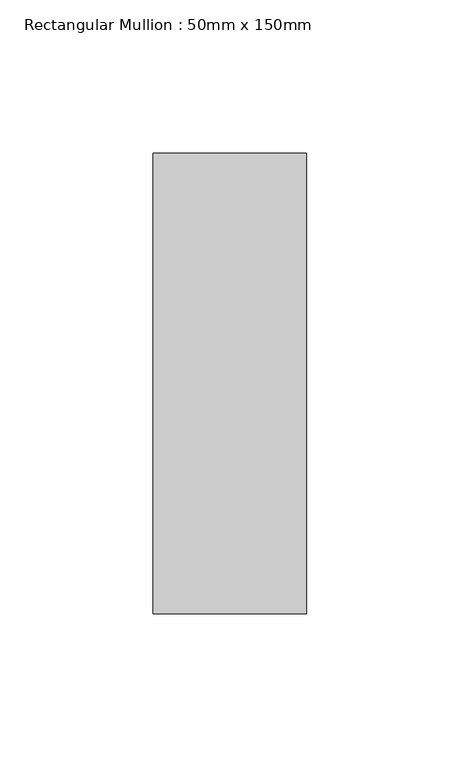
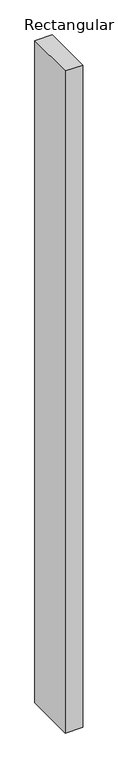
"""IFC4 building model written with IfcOpenShell, lengths in millimetres: member geometry, Rectangular Mullion : 50mm x 150mm."""

import ifcopenshell
import ifcopenshell.guid

model = None  # the IFC model being written
_history = None  # IfcOwnerHistory: only IFC2X3 demands one
_inside = {}  # id of a spatial element -> (the spatial element, [elements in it])
_under = {}  # id of a project, library or spatial element -> (it, [spatial elements below it])
_declared = {}  # id of a project -> (the project, [libraries it declares])
_typed = {}  # id of a type object -> (the type object, [elements of that type])
_made_of = {}  # id of a material, layer set ... -> (it, [elements and type objects made of it])


def new_model(schema):
    """Start an empty IFC model of exactly this schema.

    Asked for "IFC4X3", IfcOpenShell would pick the latest addendum, in which some entities
    have other attributes; the version numbers below select the first issue.
    IFC2X3 requires an IfcOwnerHistory on every rooted entity: one is made here for all.
    """
    global model, _history
    if schema == "IFC4X3":
        model = ifcopenshell.file(schema_version=(4, 3, 0, 0))
    else:
        model = ifcopenshell.file(schema=schema)
    _inside.clear()
    _under.clear()
    _declared.clear()
    _typed.clear()
    _made_of.clear()
    _history = None
    if model.schema == "IFC2X3":
        org = make("IfcOrganization", Name="unknown")
        user = make(
            "IfcPersonAndOrganization",
            ThePerson=make("IfcPerson", FamilyName="unknown"),
            TheOrganization=org,
        )
        app = make(
            "IfcApplication",
            ApplicationDeveloper=org,
            Version="unknown",
            ApplicationFullName="unknown",
            ApplicationIdentifier="unknown",
        )
        _history = make(
            "IfcOwnerHistory",
            OwningUser=user,
            OwningApplication=app,
            ChangeAction="ADDED",
            CreationDate=0,
        )
    return model


def make(cls, **values):
    """One entity of the class cls with the attributes given. An attribute that is None is left unset."""
    return model.create_entity(
        cls, **{name: value for name, value in values.items() if value is not None}
    )


def rooted(cls, **values):
    """An entity with a GlobalId (a new one), such as an element, a storey or a relation."""
    return make(cls, GlobalId=ifcopenshell.guid.new(), OwnerHistory=_history, **values)


def si_unit(unit_type, name, prefix=None):
    """IfcSIUnit, for example si_unit("LENGTHUNIT", "METRE", prefix="MILLI")."""
    return make("IfcSIUnit", UnitType=unit_type, Prefix=prefix, Name=name)


def assignment(units):
    """IfcUnitAssignment: the units of a project."""
    return None if units is None else make("IfcUnitAssignment", Units=units)


def point(xyz):
    """IfcCartesianPoint."""
    return None if xyz is None else make("IfcCartesianPoint", Coordinates=xyz)


def direction(xyz):
    """IfcDirection."""
    return None if xyz is None else make("IfcDirection", DirectionRatios=xyz)


def frame(location, z_axis=None, x_axis=None):
    """IfcAxis2Placement3D, a coordinate frame: its origin and axes. An axis left out is left unset."""
    return make(
        "IfcAxis2Placement3D",
        Location=point(location),
        Axis=direction(z_axis),
        RefDirection=direction(x_axis),
    )


def origin():
    """The frame at (0, 0, 0) with its axes left unset."""
    return frame((0.0, 0.0, 0.0))


def place(relative_to, where):
    """IfcLocalPlacement: puts the frame where relative to a parent placement (None: the world)."""
    return make(
        "IfcLocalPlacement", PlacementRelTo=relative_to, RelativePlacement=where
    )


def context(
    kind, dimensions, precision=None, world=None, true_north=None, identifier=None
):
    """IfcGeometricRepresentationContext, for example the 3D "Model" context."""
    return make(
        "IfcGeometricRepresentationContext",
        ContextIdentifier=identifier,
        ContextType=kind,
        CoordinateSpaceDimension=dimensions,
        Precision=precision,
        WorldCoordinateSystem=world,
        TrueNorth=true_north,
    )


def project(units=None, contexts=None):
    """IfcProject with its units and contexts."""
    return rooted(
        "IfcProject",
        Name="project",
        RepresentationContexts=contexts,
        UnitsInContext=assignment(units),
    )


def spatial(cls, under=None, at=None, **own):
    """A site, building, storey or space (cls), placed at a placement, below another one or the project."""
    s = rooted(cls, ObjectPlacement=at, **own)
    if under is not None:
        _under.setdefault(under.id(), (under, []))[1].append(s)
    return s


def polyline(points):
    """IfcPolyline through the points."""
    return make("IfcPolyline", Points=[point(p) for p in points])


def outline(outer, holes=None, kind="AREA"):
    """IfcArbitraryClosedProfileDef: a profile drawn as a closed curve; with holes, ...WithVoids."""
    if holes is None:
        return make("IfcArbitraryClosedProfileDef", ProfileType=kind, OuterCurve=outer)
    return make(
        "IfcArbitraryProfileDefWithVoids",
        ProfileType=kind,
        OuterCurve=outer,
        InnerCurves=holes,
    )


def extrude(swept, where, along, depth):
    """IfcExtrudedAreaSolid: the profile swept, set in the frame where, extruded along a direction by depth."""
    return make(
        "IfcExtrudedAreaSolid",
        SweptArea=swept,
        Position=where,
        ExtrudedDirection=direction(along),
        Depth=depth,
    )


def shape(context_of_items, identifier, shape_type, items):
    """IfcShapeRepresentation: the items that make up one representation, for example the "Body"."""
    return make(
        "IfcShapeRepresentation",
        ContextOfItems=context_of_items,
        RepresentationIdentifier=identifier,
        RepresentationType=shape_type,
        Items=items,
    )


def source(mapping_origin, context_of_items, identifier, shape_type, items):
    """IfcRepresentationMap: a shape defined once, which mapped items show again and again."""
    return make(
        "IfcRepresentationMap",
        MappingOrigin=mapping_origin,
        MappedRepresentation=shape(context_of_items, identifier, shape_type, items),
    )


def transform(
    local_origin,
    x_axis=None,
    y_axis=None,
    z_axis=None,
    scale=None,
    scale2=None,
    scale3=None,
    uniform=True,
):
    """IfcCartesianTransformationOperator3D, or its non-uniform kind. x_axis, y_axis, z_axis: its Axis1, 2, 3."""
    if uniform:
        return make(
            "IfcCartesianTransformationOperator3D",
            Axis1=direction(x_axis),
            Axis2=direction(y_axis),
            LocalOrigin=point(local_origin),
            Scale=scale,
            Axis3=direction(z_axis),
        )
    return make(
        "IfcCartesianTransformationOperator3DnonUniform",
        Axis1=direction(x_axis),
        Axis2=direction(y_axis),
        LocalOrigin=point(local_origin),
        Scale=scale,
        Axis3=direction(z_axis),
        Scale2=scale2,
        Scale3=scale3,
    )


def mapped(mapping_source, mapping_target):
    """IfcMappedItem: shows the shape of a source again, moved by a transform."""
    return make(
        "IfcMappedItem", MappingSource=mapping_source, MappingTarget=mapping_target
    )


def made_of(thing, what):
    """Note that an element or type object is made of a material, layer set ...; save() writes the relation."""
    if what is not None:
        _made_of.setdefault(what.id(), (what, []))[1].append(thing)
    return thing


def element(
    cls,
    number,
    at=None,
    inside=None,
    cuts=None,
    type_object=None,
    material=None,
    context=None,
    identifier="Body",
    shape_type=None,
    held_by="IfcProductDefinitionShape",
    body=None,
    shapes=None,
    **own,
):
    """One element of the class cls, such as IfcWall. Its Tag is "e" and its number.

    at: its placement. inside: the storey or other place that contains it. cuts: it is an
    opening in that element (IfcRelVoidsElement). A single representation is given by context,
    identifier, shape_type and body (its items); several are given by shapes. held_by: the class
    of the entity that holds the representations. save() writes the other relations.
    """
    e = rooted(cls, Tag="e%d" % number, ObjectPlacement=at, **own)
    if body is not None:
        shapes = [shape(context, identifier, shape_type, body)]
    if shapes is not None:
        e.Representation = make(held_by, Representations=shapes)
    if inside is not None:
        _inside.setdefault(inside.id(), (inside, []))[1].append(e)
    if cuts is not None:
        rooted(
            "IfcRelVoidsElement", RelatingBuildingElement=cuts, RelatedOpeningElement=e
        )
    if type_object is not None:
        _typed.setdefault(type_object.id(), (type_object, []))[1].append(e)
    return made_of(e, material)


def aggregate(whole, parts):
    """IfcRelAggregates: a whole, such as a stair, and the parts it consists of."""
    return rooted("IfcRelAggregates", RelatingObject=whole, RelatedObjects=parts)


def save(model, path):
    """Write the relations noted so far, then the file.

    IfcRelAggregates (storeys below a building ...), IfcRelContainedInSpatialStructure (elements
    in a storey), IfcRelDefinesByType, IfcRelAssociatesMaterial and IfcRelDeclares: one each for
    every whole, place, type object, material and project.
    """
    for whole, parts in _under.values():
        aggregate(whole, parts)
    for where, things in _inside.values():
        rooted(
            "IfcRelContainedInSpatialStructure",
            RelatedElements=things,
            RelatingStructure=where,
        )
    for kind, things in _typed.values():
        rooted("IfcRelDefinesByType", RelatedObjects=things, RelatingType=kind)
    for what, things in _made_of.values():
        rooted("IfcRelAssociatesMaterial", RelatedObjects=things, RelatingMaterial=what)
    for by, libraries in _declared.values():
        rooted("IfcRelDeclares", RelatingContext=by, RelatedDefinitions=libraries)
    model.write(path)


def rectangular_mullion_50mm_x_150mm_aa47fe12(model_context):
    return source(origin(), model_context, "Body", "SweptSolid", [
        extrude(outline(polyline([(0.0, 75.0), (0.0, -75.0), (-50.0, -75.0), (-50.0, 75.0), (0.0, 75.0)])), frame((0.0, 0.0, -2000.0), z_axis=(0.0, 0.0, 1.0), x_axis=(1.0, 0.0, 0.0)), (0.0, 0.0, 1.0), 2000.0),
    ])


if __name__ == "__main__":
    model = new_model("IFC4")
    model_context = context("Model", 3, world=origin())
    ifc_project = project(units=[si_unit("LENGTHUNIT", "METRE", prefix="MILLI")], contexts=[model_context])
    site = spatial("IfcSite", under=ifc_project)
    building = spatial("IfcBuilding", under=site)
    placement = place(None, origin())
    rectangular_mullion_50mm_x_150mm_shape = rectangular_mullion_50mm_x_150mm_aa47fe12(model_context)
    element("IfcMember", 1, ObjectType="Rectangular Mullion : 50mm x 150mm", at=placement, inside=building, context=model_context, shape_type="MappedRepresentation", body=[
        mapped(rectangular_mullion_50mm_x_150mm_shape, transform((0.0, 0.0, 0.0), x_axis=(1.0, 0.0, 0.0), y_axis=(0.0, 1.0, 0.0), z_axis=(0.0, 0.0, 1.0))),
    ])
    save(model, "model.ifc")

# Revit data of these elements
# Type "Rectangular Mullion : 50mm x 150mm"
#   built-in parameter 1007304 = 0.492126 (stored number, unit not read)
#   built-in parameter 1007301 = 0.082021 (stored number, unit not read)
#   built-in parameter 1007300 = 0.082021 (stored number, unit not read)
# Element 1 (IfcMember, "Rectangular Mullion : 50mm x 150mm")
#   Materials on its faces: "Aluminum"
# Materials
#   "Aluminum": class "Metal", colour RGB 244 244 244, transparency 0, Description = "Aluminum 6061", Cost = 0
